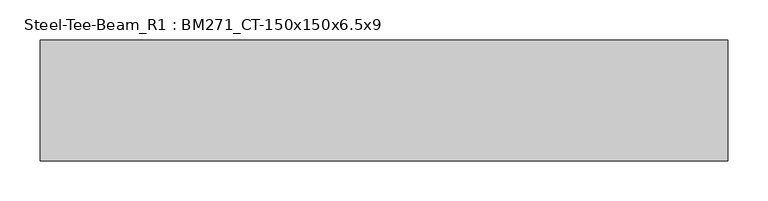
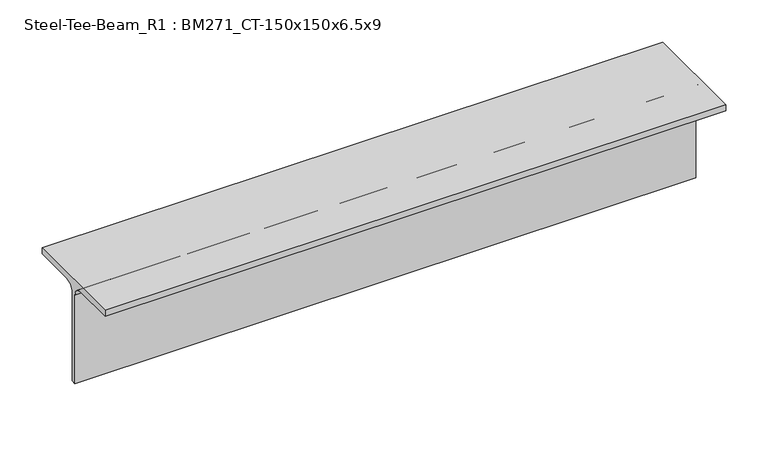
"""IFC4 building model written with IfcOpenShell, lengths in millimetres: member geometry, Steel-Tee-Beam_R1 : BM271_CT-150x150x6.5x9."""

import ifcopenshell
import ifcopenshell.guid

model = None  # the IFC model being written
_history = None  # IfcOwnerHistory: only IFC2X3 demands one
_inside = {}  # id of a spatial element -> (the spatial element, [elements in it])
_under = {}  # id of a project, library or spatial element -> (it, [spatial elements below it])
_declared = {}  # id of a project -> (the project, [libraries it declares])
_typed = {}  # id of a type object -> (the type object, [elements of that type])
_made_of = {}  # id of a material, layer set ... -> (it, [elements and type objects made of it])


def new_model(schema):
    """Start an empty IFC model of exactly this schema.

    Asked for "IFC4X3", IfcOpenShell would pick the latest addendum, in which some entities
    have other attributes; the version numbers below select the first issue.
    IFC2X3 requires an IfcOwnerHistory on every rooted entity: one is made here for all.
    """
    global model, _history
    if schema == "IFC4X3":
        model = ifcopenshell.file(schema_version=(4, 3, 0, 0))
    else:
        model = ifcopenshell.file(schema=schema)
    _inside.clear()
    _under.clear()
    _declared.clear()
    _typed.clear()
    _made_of.clear()
    _history = None
    if model.schema == "IFC2X3":
        org = make("IfcOrganization", Name="unknown")
        user = make(
            "IfcPersonAndOrganization",
            ThePerson=make("IfcPerson", FamilyName="unknown"),
            TheOrganization=org,
        )
        app = make(
            "IfcApplication",
            ApplicationDeveloper=org,
            Version="unknown",
            ApplicationFullName="unknown",
            ApplicationIdentifier="unknown",
        )
        _history = make(
            "IfcOwnerHistory",
            OwningUser=user,
            OwningApplication=app,
            ChangeAction="ADDED",
            CreationDate=0,
        )
    return model


def make(cls, **values):
    """One entity of the class cls with the attributes given. An attribute that is None is left unset."""
    return model.create_entity(
        cls, **{name: value for name, value in values.items() if value is not None}
    )


def rooted(cls, **values):
    """An entity with a GlobalId (a new one), such as an element, a storey or a relation."""
    return make(cls, GlobalId=ifcopenshell.guid.new(), OwnerHistory=_history, **values)


def si_unit(unit_type, name, prefix=None):
    """IfcSIUnit, for example si_unit("LENGTHUNIT", "METRE", prefix="MILLI")."""
    return make("IfcSIUnit", UnitType=unit_type, Prefix=prefix, Name=name)


def assignment(units):
    """IfcUnitAssignment: the units of a project."""
    return None if units is None else make("IfcUnitAssignment", Units=units)


def point(xyz):
    """IfcCartesianPoint."""
    return None if xyz is None else make("IfcCartesianPoint", Coordinates=xyz)


def direction(xyz):
    """IfcDirection."""
    return None if xyz is None else make("IfcDirection", DirectionRatios=xyz)


def frame(location, z_axis=None, x_axis=None):
    """IfcAxis2Placement3D, a coordinate frame: its origin and axes. An axis left out is left unset."""
    return make(
        "IfcAxis2Placement3D",
        Location=point(location),
        Axis=direction(z_axis),
        RefDirection=direction(x_axis),
    )


def frame_2d(location, x_axis=None):
    """IfcAxis2Placement2D, a coordinate frame in the plane: its origin and x axis."""
    return make(
        "IfcAxis2Placement2D", Location=point(location), RefDirection=direction(x_axis)
    )


def origin():
    """The frame at (0, 0, 0) with its axes left unset."""
    return frame((0.0, 0.0, 0.0))


def place(relative_to, where):
    """IfcLocalPlacement: puts the frame where relative to a parent placement (None: the world)."""
    return make(
        "IfcLocalPlacement", PlacementRelTo=relative_to, RelativePlacement=where
    )


def context(
    kind, dimensions, precision=None, world=None, true_north=None, identifier=None
):
    """IfcGeometricRepresentationContext, for example the 3D "Model" context."""
    return make(
        "IfcGeometricRepresentationContext",
        ContextIdentifier=identifier,
        ContextType=kind,
        CoordinateSpaceDimension=dimensions,
        Precision=precision,
        WorldCoordinateSystem=world,
        TrueNorth=true_north,
    )


def project(units=None, contexts=None):
    """IfcProject with its units and contexts."""
    return rooted(
        "IfcProject",
        Name="project",
        RepresentationContexts=contexts,
        UnitsInContext=assignment(units),
    )


def spatial(cls, under=None, at=None, **own):
    """A site, building, storey or space (cls), placed at a placement, below another one or the project."""
    s = rooted(cls, ObjectPlacement=at, **own)
    if under is not None:
        _under.setdefault(under.id(), (under, []))[1].append(s)
    return s


def polyline(points):
    """IfcPolyline through the points."""
    return make("IfcPolyline", Points=[point(p) for p in points])


def circle_curve(where, radius):
    """IfcCircle in the frame where."""
    return make("IfcCircle", Position=where, Radius=radius)


def trimmed(basis, trim1, trim2, sense, master):
    """IfcTrimmedCurve: the piece of a basis curve between two trims."""
    return make(
        "IfcTrimmedCurve",
        BasisCurve=basis,
        Trim1=trim1,
        Trim2=trim2,
        SenseAgreement=sense,
        MasterRepresentation=master,
    )


def segment(curve, same_sense, transition):
    """IfcCompositeCurveSegment."""
    return make(
        "IfcCompositeCurveSegment",
        Transition=transition,
        SameSense=same_sense,
        ParentCurve=curve,
    )


def composite_curve(segments, self_intersect=None):
    """IfcCompositeCurve: segments joined end to end."""
    return make("IfcCompositeCurve", Segments=segments, SelfIntersect=self_intersect)


def outline(outer, holes=None, kind="AREA"):
    """IfcArbitraryClosedProfileDef: a profile drawn as a closed curve; with holes, ...WithVoids."""
    if holes is None:
        return make("IfcArbitraryClosedProfileDef", ProfileType=kind, OuterCurve=outer)
    return make(
        "IfcArbitraryProfileDefWithVoids",
        ProfileType=kind,
        OuterCurve=outer,
        InnerCurves=holes,
    )


def extrude(swept, where, along, depth):
    """IfcExtrudedAreaSolid: the profile swept, set in the frame where, extruded along a direction by depth."""
    return make(
        "IfcExtrudedAreaSolid",
        SweptArea=swept,
        Position=where,
        ExtrudedDirection=direction(along),
        Depth=depth,
    )


def shape(context_of_items, identifier, shape_type, items):
    """IfcShapeRepresentation: the items that make up one representation, for example the "Body"."""
    return make(
        "IfcShapeRepresentation",
        ContextOfItems=context_of_items,
        RepresentationIdentifier=identifier,
        RepresentationType=shape_type,
        Items=items,
    )


def source(mapping_origin, context_of_items, identifier, shape_type, items):
    """IfcRepresentationMap: a shape defined once, which mapped items show again and again."""
    return make(
        "IfcRepresentationMap",
        MappingOrigin=mapping_origin,
        MappedRepresentation=shape(context_of_items, identifier, shape_type, items),
    )


def transform(
    local_origin,
    x_axis=None,
    y_axis=None,
    z_axis=None,
    scale=None,
    scale2=None,
    scale3=None,
    uniform=True,
):
    """IfcCartesianTransformationOperator3D, or its non-uniform kind. x_axis, y_axis, z_axis: its Axis1, 2, 3."""
    if uniform:
        return make(
            "IfcCartesianTransformationOperator3D",
            Axis1=direction(x_axis),
            Axis2=direction(y_axis),
            LocalOrigin=point(local_origin),
            Scale=scale,
            Axis3=direction(z_axis),
        )
    return make(
        "IfcCartesianTransformationOperator3DnonUniform",
        Axis1=direction(x_axis),
        Axis2=direction(y_axis),
        LocalOrigin=point(local_origin),
        Scale=scale,
        Axis3=direction(z_axis),
        Scale2=scale2,
        Scale3=scale3,
    )


def mapped(mapping_source, mapping_target):
    """IfcMappedItem: shows the shape of a source again, moved by a transform."""
    return make(
        "IfcMappedItem", MappingSource=mapping_source, MappingTarget=mapping_target
    )


def made_of(thing, what):
    """Note that an element or type object is made of a material, layer set ...; save() writes the relation."""
    if what is not None:
        _made_of.setdefault(what.id(), (what, []))[1].append(thing)
    return thing


def element(
    cls,
    number,
    at=None,
    inside=None,
    cuts=None,
    type_object=None,
    material=None,
    context=None,
    identifier="Body",
    shape_type=None,
    held_by="IfcProductDefinitionShape",
    body=None,
    shapes=None,
    **own,
):
    """One element of the class cls, such as IfcWall. Its Tag is "e" and its number.

    at: its placement. inside: the storey or other place that contains it. cuts: it is an
    opening in that element (IfcRelVoidsElement). A single representation is given by context,
    identifier, shape_type and body (its items); several are given by shapes. held_by: the class
    of the entity that holds the representations. save() writes the other relations.
    """
    e = rooted(cls, Tag="e%d" % number, ObjectPlacement=at, **own)
    if body is not None:
        shapes = [shape(context, identifier, shape_type, body)]
    if shapes is not None:
        e.Representation = make(held_by, Representations=shapes)
    if inside is not None:
        _inside.setdefault(inside.id(), (inside, []))[1].append(e)
    if cuts is not None:
        rooted(
            "IfcRelVoidsElement", RelatingBuildingElement=cuts, RelatedOpeningElement=e
        )
    if type_object is not None:
        _typed.setdefault(type_object.id(), (type_object, []))[1].append(e)
    return made_of(e, material)


def aggregate(whole, parts):
    """IfcRelAggregates: a whole, such as a stair, and the parts it consists of."""
    return rooted("IfcRelAggregates", RelatingObject=whole, RelatedObjects=parts)


def save(model, path):
    """Write the relations noted so far, then the file.

    IfcRelAggregates (storeys below a building ...), IfcRelContainedInSpatialStructure (elements
    in a storey), IfcRelDefinesByType, IfcRelAssociatesMaterial and IfcRelDeclares: one each for
    every whole, place, type object, material and project.
    """
    for whole, parts in _under.values():
        aggregate(whole, parts)
    for where, things in _inside.values():
        rooted(
            "IfcRelContainedInSpatialStructure",
            RelatedElements=things,
            RelatingStructure=where,
        )
    for kind, things in _typed.values():
        rooted("IfcRelDefinesByType", RelatedObjects=things, RelatingType=kind)
    for what, things in _made_of.values():
        rooted("IfcRelAssociatesMaterial", RelatedObjects=things, RelatingMaterial=what)
    for by, libraries in _declared.values():
        rooted("IfcRelDeclares", RelatingContext=by, RelatedDefinitions=libraries)
    model.write(path)


def steel_tee_beam_r1_bm271_ct_150x150x6_5x9_d8092f7d(model_context):
    return source(origin(), model_context, "Body", "SweptSolid", [
        extrude(outline(composite_curve([segment(polyline([(75.0, 75.0), (75.0, 66.0), (16.25, 66.0)]), True, "CONTINUOUS"), segment(trimmed(circle_curve(frame_2d((16.25, 53.0)), 13.0), [point((16.25, 66.0))], [point((3.25, 53.0))], True, "CARTESIAN"), True, "CONTINUOUS"), segment(polyline([(3.25, 53.0), (3.25, -75.0), (-3.25, -75.0), (-3.25, 53.0)]), True, "CONTINUOUS"), segment(trimmed(circle_curve(frame_2d((-16.25, 53.0)), 13.0), [point((-3.25, 53.0))], [point((-16.25, 66.0))], True, "CARTESIAN"), True, "CONTINUOUS"), segment(polyline([(-16.25, 66.0), (-75.0, 66.0), (-75.0, 75.0), (75.0, 75.0)]), True, "CONTINUOUS")], self_intersect=False)), frame((-353.0826681, 0.0, 0.0), z_axis=(1.0, 0.0, 0.0), x_axis=(0.0, 1.0, 0.0)), (0.0, 0.0, 1.0), 853.0826681),
    ])


if __name__ == "__main__":
    model = new_model("IFC4")
    model_context = context("Model", 3, world=origin())
    ifc_project = project(units=[si_unit("LENGTHUNIT", "METRE", prefix="MILLI")], contexts=[model_context])
    site = spatial("IfcSite", under=ifc_project)
    building = spatial("IfcBuilding", under=site)
    placement = place(None, origin())
    steel_tee_beam_r1_bm271_ct_150x150x6_5x9_shape = steel_tee_beam_r1_bm271_ct_150x150x6_5x9_d8092f7d(model_context)
    element("IfcMember", 1, ObjectType="Steel-Tee-Beam_R1 : BM271_CT-150x150x6.5x9", at=placement, inside=building, context=model_context, shape_type="MappedRepresentation", body=[
        mapped(steel_tee_beam_r1_bm271_ct_150x150x6_5x9_shape, transform((0.0, 0.0, 0.0), x_axis=(1.0, 0.0, 0.0), y_axis=(0.0, 1.0, 0.0), z_axis=(0.0, 0.0, 1.0))),
    ])
    save(model, "model.ifc")

# Revit data of these elements
# Type "Steel-Tee-Beam_R1 : BM271_CT-150x150x6.5x9"
#   Keynote = "CT-150x150x6.5x9"
#   Surface Area = 0.588841 m²/m
#   Section Area = 23.3904 cm²
#   Mass per Unit Length = 18.3614 kg/m
#   Length [instance default] = 1.5240 m
#   bf = 0.1500 m
#   d = 0.1500 m
#   k = 0.0220 m
#   r = 0.0130 m
#   tf = 0.0090 m
#   tw = 0.0065 m
#   hec_material4 [instance default] = none
#   hec_material3 [instance default] = none
#   hec_material2 [instance default] = none
#   hec_material1 [instance default] = none
#   Structural Material [instance default] = Steel, 45-345
#   Assembly Code = ""
# Element 1 (IfcMember, "Steel-Tee-Beam_R1 : BM271_CT-150x150x6.5x9")
#   Structural Material = none
# Materials
#   "Steel, 45-345": class "Metal", colour RGB 189 187 185, transparency 0, Description = "Steel 345 MPa", Cost = 0
